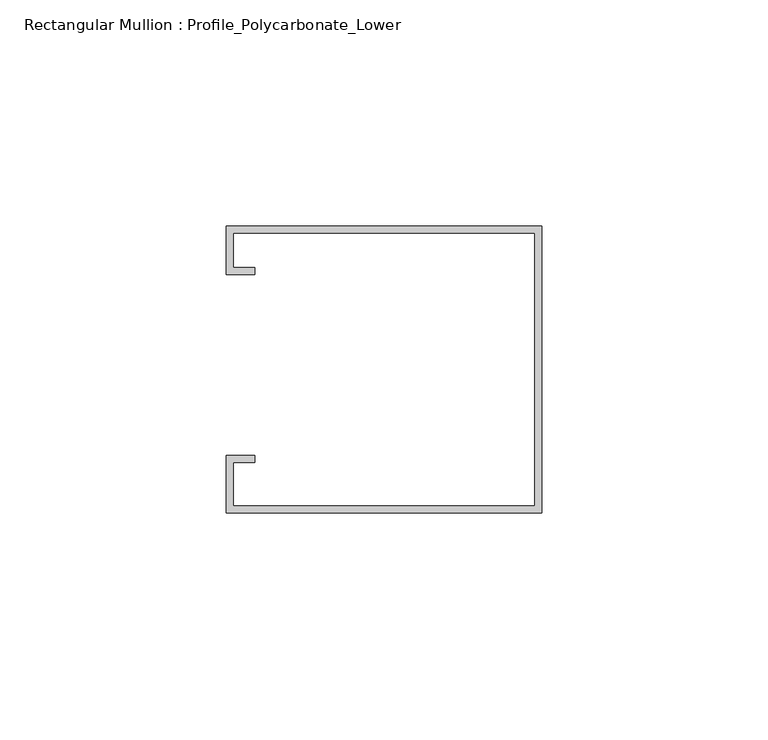
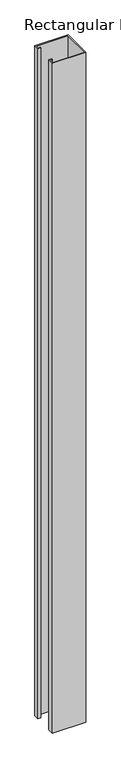
"""IFC4 building model written with IfcOpenShell, lengths in millimetres: member geometry, Rectangular Mullion : Profile_Polycarbonate_Lower."""

from ifc_helpers import new_model, si_unit, frame, origin, place, context, project, spatial, polyline, outline, extrude, source, transform, mapped, element, save


def rectangular_mullion_profile_polycarbonate_lower_0e7361e1(model_context):
    return source(origin(), model_context, "Body", "SweptSolid", [
        extrude(outline(polyline([(0.0, -32.7), (-69.85, -32.7), (-69.85, -20.0), (-63.5, -20.0), (-63.5, -21.5875), (-68.2625, -21.5875), (-68.2625, -31.1125), (-1.5875, -31.1125), (-1.5875, 29.2125), (-68.2625, 29.2125), (-68.2625, 21.5875), (-63.5, 21.5875), (-63.5, 20.0), (-69.85, 20.0), (-69.85, 30.8), (0.0, 30.8), (0.0, -32.7)])), frame((0.0, 0.0, -1481.775), z_axis=(0.0, 0.0, 1.0), x_axis=(1.0, 0.0, 0.0)), (0.0, 0.0, 1.0), 1481.775),
    ])


if __name__ == "__main__":
    model = new_model("IFC4")
    model_context = context("Model", 3, world=origin())
    ifc_project = project(units=[si_unit("LENGTHUNIT", "METRE", prefix="MILLI")], contexts=[model_context])
    site = spatial("IfcSite", under=ifc_project)
    building = spatial("IfcBuilding", under=site)
    placement = place(None, origin())
    rectangular_mullion_profile_polycarbonate_lower_shape = rectangular_mullion_profile_polycarbonate_lower_0e7361e1(model_context)
    element("IfcMember", 1, ObjectType="Rectangular Mullion : Profile_Polycarbonate_Lower", at=placement, inside=building, context=model_context, shape_type="MappedRepresentation", body=[
        mapped(rectangular_mullion_profile_polycarbonate_lower_shape, transform((0.0, 0.0, 0.0), x_axis=(1.0, 0.0, 0.0), y_axis=(0.0, 1.0, 0.0), z_axis=(0.0, 0.0, 1.0))),
    ])
    save(model, "model.ifc")

# Revit data of these elements
# Type "Rectangular Mullion : Profile_Polycarbonate_Lower"
#   built-in parameter 1007322 = 0.208333 (stored number, unit not read)
#   built-in parameter 1007321 = 0 (stored number, unit not read)
#   built-in parameter 1007320 = 0.00520833 (stored number, unit not read)
# Element 1 (IfcMember, "Rectangular Mullion : Profile_Polycarbonate_Lower")
#   Materials on its faces: "ALUMINUM PROFILE AT POLYCARBONATE PANEL"
# Materials
#   "ALUMINUM PROFILE AT POLYCARBONATE PANEL": class "Metal", colour RGB 244 244 244, transparency 0, Description = "Aluminum 6061", Cost = 0
